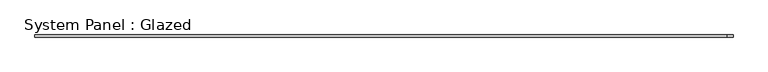
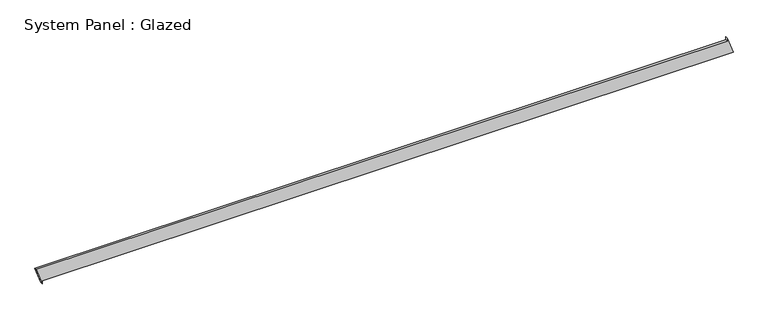
"""IFC4 building model written with IfcOpenShell, lengths in millimetres: plate geometry, System Panel : Glazed."""

from ifc_helpers import new_model, si_unit, frame, origin, place, context, project, spatial, polyline, outline, extrude, source, transform, mapped, element, save


def system_panel_glazed_38c3c94b(model_context):
    return source(origin(), model_context, "Body", "SweptSolid", [
        extrude(outline(polyline([(0.0, -3958.8254362), (35.3553391, -3958.8254362), (35.3553391, 4027.6368042), (234.820266, 3959.126507), (199.4649269, 3959.127058), (199.3404739, -4027.6368042), (0.0, -3958.8254362)])), frame((0.0, -49.5, 0.0), z_axis=(0.0, 1.0, 0.0), x_axis=(0.0, 0.0, 1.0)), (0.0, 0.0, 1.0), 25.0),
    ])


if __name__ == "__main__":
    model = new_model("IFC4")
    model_context = context("Model", 3, world=origin())
    ifc_project = project(units=[si_unit("LENGTHUNIT", "METRE", prefix="MILLI")], contexts=[model_context])
    site = spatial("IfcSite", under=ifc_project)
    building = spatial("IfcBuilding", under=site)
    placement = place(None, origin())
    system_panel_glazed_shape = system_panel_glazed_38c3c94b(model_context)
    element("IfcPlate", 1, ObjectType="System Panel : Glazed", at=placement, inside=building, context=model_context, shape_type="MappedRepresentation", body=[
        mapped(system_panel_glazed_shape, transform((0.0, 0.0, 0.0), x_axis=(1.0, 0.0, 0.0), y_axis=(0.0, 1.0, 0.0), z_axis=(0.0, 0.0, 1.0))),
    ])
    save(model, "model.ifc")

# Revit data of these elements
# Element 1 (IfcPlate, "System Panel : Glazed")
#   Materials on its faces: "Glass"
# Materials
#   "Glass": class "Glass", colour RGB 218 227 224, transparency 0.85, Description = "Soda Lime Glass", Cost = 0
